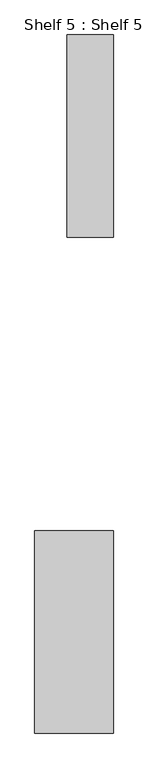
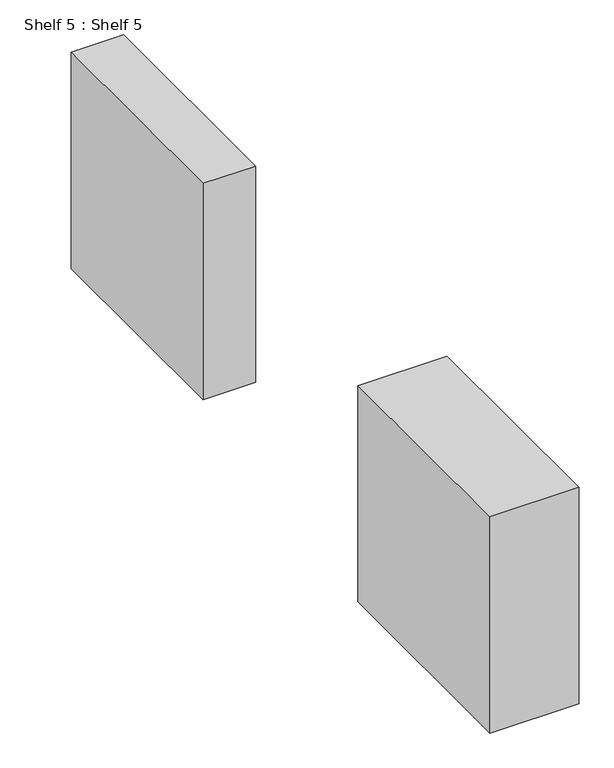
"""IFC4 building model written with IfcOpenShell, lengths in millimetres: furniture geometry, Shelf 5 : Shelf 5."""

import ifcopenshell
import ifcopenshell.guid

model = None  # the IFC model being written
_history = None  # IfcOwnerHistory: only IFC2X3 demands one
_inside = {}  # id of a spatial element -> (the spatial element, [elements in it])
_under = {}  # id of a project, library or spatial element -> (it, [spatial elements below it])
_declared = {}  # id of a project -> (the project, [libraries it declares])
_typed = {}  # id of a type object -> (the type object, [elements of that type])
_made_of = {}  # id of a material, layer set ... -> (it, [elements and type objects made of it])


def new_model(schema):
    """Start an empty IFC model of exactly this schema.

    Asked for "IFC4X3", IfcOpenShell would pick the latest addendum, in which some entities
    have other attributes; the version numbers below select the first issue.
    IFC2X3 requires an IfcOwnerHistory on every rooted entity: one is made here for all.
    """
    global model, _history
    if schema == "IFC4X3":
        model = ifcopenshell.file(schema_version=(4, 3, 0, 0))
    else:
        model = ifcopenshell.file(schema=schema)
    _inside.clear()
    _under.clear()
    _declared.clear()
    _typed.clear()
    _made_of.clear()
    _history = None
    if model.schema == "IFC2X3":
        org = make("IfcOrganization", Name="unknown")
        user = make(
            "IfcPersonAndOrganization",
            ThePerson=make("IfcPerson", FamilyName="unknown"),
            TheOrganization=org,
        )
        app = make(
            "IfcApplication",
            ApplicationDeveloper=org,
            Version="unknown",
            ApplicationFullName="unknown",
            ApplicationIdentifier="unknown",
        )
        _history = make(
            "IfcOwnerHistory",
            OwningUser=user,
            OwningApplication=app,
            ChangeAction="ADDED",
            CreationDate=0,
        )
    return model


def make(cls, **values):
    """One entity of the class cls with the attributes given. An attribute that is None is left unset."""
    return model.create_entity(
        cls, **{name: value for name, value in values.items() if value is not None}
    )


def rooted(cls, **values):
    """An entity with a GlobalId (a new one), such as an element, a storey or a relation."""
    return make(cls, GlobalId=ifcopenshell.guid.new(), OwnerHistory=_history, **values)


def si_unit(unit_type, name, prefix=None):
    """IfcSIUnit, for example si_unit("LENGTHUNIT", "METRE", prefix="MILLI")."""
    return make("IfcSIUnit", UnitType=unit_type, Prefix=prefix, Name=name)


def assignment(units):
    """IfcUnitAssignment: the units of a project."""
    return None if units is None else make("IfcUnitAssignment", Units=units)


def point(xyz):
    """IfcCartesianPoint."""
    return None if xyz is None else make("IfcCartesianPoint", Coordinates=xyz)


def direction(xyz):
    """IfcDirection."""
    return None if xyz is None else make("IfcDirection", DirectionRatios=xyz)


def frame(location, z_axis=None, x_axis=None):
    """IfcAxis2Placement3D, a coordinate frame: its origin and axes. An axis left out is left unset."""
    return make(
        "IfcAxis2Placement3D",
        Location=point(location),
        Axis=direction(z_axis),
        RefDirection=direction(x_axis),
    )


def origin():
    """The frame at (0, 0, 0) with its axes left unset."""
    return frame((0.0, 0.0, 0.0))


def origin_with_axes():
    """The frame at (0, 0, 0) with the z axis (0, 0, 1) and the x axis (1, 0, 0) written out."""
    return frame((0.0, 0.0, 0.0), z_axis=(0.0, 0.0, 1.0), x_axis=(1.0, 0.0, 0.0))


def place(relative_to, where):
    """IfcLocalPlacement: puts the frame where relative to a parent placement (None: the world)."""
    return make(
        "IfcLocalPlacement", PlacementRelTo=relative_to, RelativePlacement=where
    )


def context(
    kind, dimensions, precision=None, world=None, true_north=None, identifier=None
):
    """IfcGeometricRepresentationContext, for example the 3D "Model" context."""
    return make(
        "IfcGeometricRepresentationContext",
        ContextIdentifier=identifier,
        ContextType=kind,
        CoordinateSpaceDimension=dimensions,
        Precision=precision,
        WorldCoordinateSystem=world,
        TrueNorth=true_north,
    )


def project(units=None, contexts=None):
    """IfcProject with its units and contexts."""
    return rooted(
        "IfcProject",
        Name="project",
        RepresentationContexts=contexts,
        UnitsInContext=assignment(units),
    )


def spatial(cls, under=None, at=None, **own):
    """A site, building, storey or space (cls), placed at a placement, below another one or the project."""
    s = rooted(cls, ObjectPlacement=at, **own)
    if under is not None:
        _under.setdefault(under.id(), (under, []))[1].append(s)
    return s


def polyline(points):
    """IfcPolyline through the points."""
    return make("IfcPolyline", Points=[point(p) for p in points])


def outline(outer, holes=None, kind="AREA"):
    """IfcArbitraryClosedProfileDef: a profile drawn as a closed curve; with holes, ...WithVoids."""
    if holes is None:
        return make("IfcArbitraryClosedProfileDef", ProfileType=kind, OuterCurve=outer)
    return make(
        "IfcArbitraryProfileDefWithVoids",
        ProfileType=kind,
        OuterCurve=outer,
        InnerCurves=holes,
    )


def extrude(swept, where, along, depth):
    """IfcExtrudedAreaSolid: the profile swept, set in the frame where, extruded along a direction by depth."""
    return make(
        "IfcExtrudedAreaSolid",
        SweptArea=swept,
        Position=where,
        ExtrudedDirection=direction(along),
        Depth=depth,
    )


def shape(context_of_items, identifier, shape_type, items):
    """IfcShapeRepresentation: the items that make up one representation, for example the "Body"."""
    return make(
        "IfcShapeRepresentation",
        ContextOfItems=context_of_items,
        RepresentationIdentifier=identifier,
        RepresentationType=shape_type,
        Items=items,
    )


def source(mapping_origin, context_of_items, identifier, shape_type, items):
    """IfcRepresentationMap: a shape defined once, which mapped items show again and again."""
    return make(
        "IfcRepresentationMap",
        MappingOrigin=mapping_origin,
        MappedRepresentation=shape(context_of_items, identifier, shape_type, items),
    )


def transform(
    local_origin,
    x_axis=None,
    y_axis=None,
    z_axis=None,
    scale=None,
    scale2=None,
    scale3=None,
    uniform=True,
):
    """IfcCartesianTransformationOperator3D, or its non-uniform kind. x_axis, y_axis, z_axis: its Axis1, 2, 3."""
    if uniform:
        return make(
            "IfcCartesianTransformationOperator3D",
            Axis1=direction(x_axis),
            Axis2=direction(y_axis),
            LocalOrigin=point(local_origin),
            Scale=scale,
            Axis3=direction(z_axis),
        )
    return make(
        "IfcCartesianTransformationOperator3DnonUniform",
        Axis1=direction(x_axis),
        Axis2=direction(y_axis),
        LocalOrigin=point(local_origin),
        Scale=scale,
        Axis3=direction(z_axis),
        Scale2=scale2,
        Scale3=scale3,
    )


def mapped(mapping_source, mapping_target):
    """IfcMappedItem: shows the shape of a source again, moved by a transform."""
    return make(
        "IfcMappedItem", MappingSource=mapping_source, MappingTarget=mapping_target
    )


def made_of(thing, what):
    """Note that an element or type object is made of a material, layer set ...; save() writes the relation."""
    if what is not None:
        _made_of.setdefault(what.id(), (what, []))[1].append(thing)
    return thing


def element(
    cls,
    number,
    at=None,
    inside=None,
    cuts=None,
    type_object=None,
    material=None,
    context=None,
    identifier="Body",
    shape_type=None,
    held_by="IfcProductDefinitionShape",
    body=None,
    shapes=None,
    **own,
):
    """One element of the class cls, such as IfcWall. Its Tag is "e" and its number.

    at: its placement. inside: the storey or other place that contains it. cuts: it is an
    opening in that element (IfcRelVoidsElement). A single representation is given by context,
    identifier, shape_type and body (its items); several are given by shapes. held_by: the class
    of the entity that holds the representations. save() writes the other relations.
    """
    e = rooted(cls, Tag="e%d" % number, ObjectPlacement=at, **own)
    if body is not None:
        shapes = [shape(context, identifier, shape_type, body)]
    if shapes is not None:
        e.Representation = make(held_by, Representations=shapes)
    if inside is not None:
        _inside.setdefault(inside.id(), (inside, []))[1].append(e)
    if cuts is not None:
        rooted(
            "IfcRelVoidsElement", RelatingBuildingElement=cuts, RelatedOpeningElement=e
        )
    if type_object is not None:
        _typed.setdefault(type_object.id(), (type_object, []))[1].append(e)
    return made_of(e, material)


def aggregate(whole, parts):
    """IfcRelAggregates: a whole, such as a stair, and the parts it consists of."""
    return rooted("IfcRelAggregates", RelatingObject=whole, RelatedObjects=parts)


def save(model, path):
    """Write the relations noted so far, then the file.

    IfcRelAggregates (storeys below a building ...), IfcRelContainedInSpatialStructure (elements
    in a storey), IfcRelDefinesByType, IfcRelAssociatesMaterial and IfcRelDeclares: one each for
    every whole, place, type object, material and project.
    """
    for whole, parts in _under.values():
        aggregate(whole, parts)
    for where, things in _inside.values():
        rooted(
            "IfcRelContainedInSpatialStructure",
            RelatedElements=things,
            RelatingStructure=where,
        )
    for kind, things in _typed.values():
        rooted("IfcRelDefinesByType", RelatedObjects=things, RelatingType=kind)
    for what, things in _made_of.values():
        rooted("IfcRelAssociatesMaterial", RelatedObjects=things, RelatingMaterial=what)
    for by, libraries in _declared.values():
        rooted("IfcRelDeclares", RelatingContext=by, RelatedDefinitions=libraries)
    model.write(path)


def shelf_5_shelf_5_5ccbb831(model_context):
    return source(origin(), model_context, "Body", "SweptSolid", [
        extrude(outline(polyline([(22771.8870052, 5354.3115366), (22561.5672994, 5354.3115366), (22561.5672994, 6268.7115366), (22771.8870052, 6268.7115366), (22771.8870052, 5354.3115366)])), origin_with_axes(), (0.0, 0.0, 1.0), 914.4),
        extrude(outline(polyline([(22771.8870052, 3112.7615366), (22416.2870052, 3112.7615366), (22416.2870052, 4027.1615366), (22771.8870052, 4027.1615366), (22771.8870052, 3112.7615366)])), origin_with_axes(), (0.0, 0.0, 1.0), 914.4),
    ])


if __name__ == "__main__":
    model = new_model("IFC4")
    model_context = context("Model", 3, world=origin())
    ifc_project = project(units=[si_unit("LENGTHUNIT", "METRE", prefix="MILLI")], contexts=[model_context])
    site = spatial("IfcSite", under=ifc_project)
    building = spatial("IfcBuilding", under=site)
    placement = place(None, origin())
    shelf_5_shelf_5_shape = shelf_5_shelf_5_5ccbb831(model_context)
    element("IfcFurniture", 1, ObjectType="Shelf 5 : Shelf 5", at=placement, inside=building, context=model_context, shape_type="MappedRepresentation", body=[
        mapped(shelf_5_shelf_5_shape, transform((0.0, 0.0, 0.0), x_axis=(1.0, 0.0, 0.0), y_axis=(0.0, 1.0, 0.0), z_axis=(0.0, 0.0, 1.0))),
    ])
    save(model, "model.ifc")

# Revit data of these elements
# Element 1 (IfcFurniture, "Shelf 5 : Shelf 5")
#   Materials on its faces: "food"
# Materials
#   "food": class "Glass", colour RGB 233 233 233, transparency 0, Description = "Soda Lime Glass", Cost = 0
